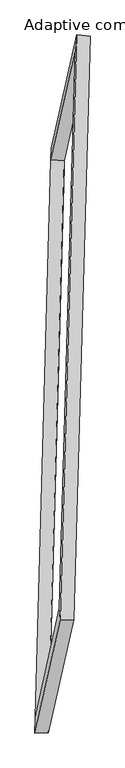
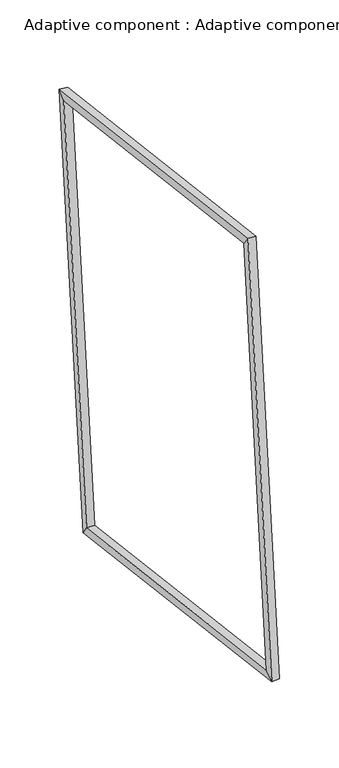
"""IFC4 building model written with IfcOpenShell, lengths in millimetres: proxy geometry, Adaptive component : Adaptive component."""

from ifc_helpers import new_model, si_unit, origin, place, context, project, spatial, faceted_brep, source, transform, mapped, element, save


def adaptive_component_adaptive_component_de21833b(model_context):
    return source(origin(), model_context, "Body", "Brep", [
        faceted_brep([(72.686125, 1184.925234, 2798.8706496), (137.3318978, 1179.0173474, 2794.1857583), (62.0725754, -1498.1704147, 3218.4456578), (-2.7566881, -1498.7898123, 3224.1649423), (80.0375192, 1259.0007043, 2852.7023729), (0.9913334, -1552.8965395, 3298.3099836), (144.683292, 1253.0928177, 2848.0174816), (65.8205968, -1552.2771419, 3292.590699), (-54.4830295, -2021.6283887, -105.382919), (-119.5411688, -2023.2756811, -106.1905117), (-120.2877901, -2097.5681091, -160.2196745), (-55.2296508, -2095.9208167, -159.4120818), (20.7762929, 655.5593734, -529.6428184), (-44.0983557, 660.4393653, -531.4848044), (-41.2416043, 714.3291348, -605.8272852), (23.6330444, 709.4491429, -603.9852992)], [[[0, 1, 2, 3]], [[4, 0, 3, 5]], [[6, 4, 5, 7]], [[1, 6, 7, 2]], [[3, 2, 8, 9]], [[5, 3, 9, 10]], [[7, 5, 10, 11]], [[2, 7, 11, 8]], [[9, 8, 12, 13]], [[10, 9, 13, 14]], [[11, 10, 14, 15]], [[8, 11, 15, 12]], [[13, 12, 1, 0]], [[14, 13, 0, 4]], [[15, 14, 4, 6]], [[12, 15, 6, 1]]]),
    ])


if __name__ == "__main__":
    model = new_model("IFC4")
    model_context = context("Model", 3, world=origin())
    ifc_project = project(units=[si_unit("LENGTHUNIT", "METRE", prefix="MILLI")], contexts=[model_context])
    site = spatial("IfcSite", under=ifc_project)
    building = spatial("IfcBuilding", under=site)
    placement = place(None, origin())
    adaptive_component_adaptive_component_shape = adaptive_component_adaptive_component_de21833b(model_context)
    element("IfcBuildingElementProxy", 1, Name="Adaptive component : Adaptive component", ObjectType="Adaptive component : Adaptive component", at=placement, inside=building, context=model_context, shape_type="MappedRepresentation", body=[
        mapped(adaptive_component_adaptive_component_shape, transform((0.0, 0.0, 0.0), x_axis=(1.0, 0.0, 0.0), y_axis=(0.0, 1.0, 0.0), z_axis=(0.0, 0.0, 1.0))),
    ])
    save(model, "model.ifc")

# Revit data of these elements
# Type "Adaptive component : Adaptive component"
#   r [instance default] = 2063.125 mm
#   2r [instance default] = 4126.251 mm
#   Number [instance default] = 5
#   Default Elevation = 0
# Element 1 (IfcBuildingElementProxy, "Adaptive component : Adaptive component")
#   r = 2255.163 mm
#   2r = 4510.326 mm
#   Number = 12
